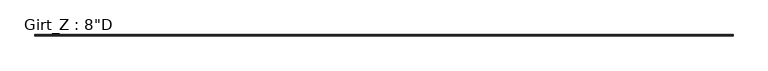
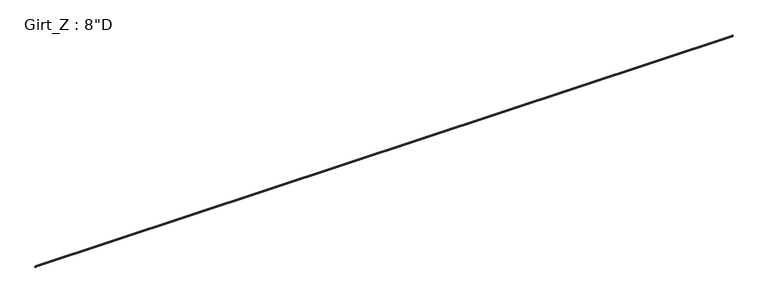
"""IFC4 building model written with IfcOpenShell, lengths in millimetres: beam geometry."""

from ifc_helpers import new_model, si_unit, point, frame, frame_2d, origin, place, context, project, spatial, polyline, circle_curve, trimmed, segment, composite_curve, outline, extrude, source, transform, mapped, element, save


def beam_4e68f0c2(model_context):
    return source(origin(), model_context, "Body", "SweptSolid", [
        extrude(outline(composite_curve([segment(polyline([(-63.5, 101.6), (-3.3734375, 101.6)]), True, "CONTINUOUS"), segment(trimmed(circle_curve(frame_2d((-3.3734375, 96.8375)), 4.7625), [point((-3.3734375, 101.6))], [point((1.3890625, 96.8375))], False, "CARTESIAN"), True, "CONTINUOUS"), segment(polyline([(1.3890625, 96.8375), (1.3890625, -96.8389339)]), True, "CONTINUOUS"), segment(trimmed(circle_curve(frame_2d((3.3748024, -96.8389339)), 1.9857399), [point((1.3890625, -96.8389339))], [point((3.2694106, -98.821875))], True, "CARTESIAN"), True, "CONTINUOUS"), segment(polyline([(3.2694106, -98.821875), (62.204539, -98.821875), (73.6169367, -85.221109), (75.745104, -87.0068534), (63.5, -101.6), (3.3734375, -101.6)]), True, "CONTINUOUS"), segment(trimmed(circle_curve(frame_2d((3.3734375, -96.8375)), 4.7625), [point((3.3734375, -101.6))], [point((-1.3890625, -96.8375))], False, "CARTESIAN"), True, "CONTINUOUS"), segment(polyline([(-1.3890625, -96.8375), (-1.3890625, 96.8381931)]), True, "CONTINUOUS"), segment(trimmed(circle_curve(frame_2d((-3.3741066, 96.8381931)), 1.9850441), [point((-1.3890625, 96.8381931))], [point((-3.3005807, 98.821875))], True, "CARTESIAN"), True, "CONTINUOUS"), segment(polyline([(-3.3005807, 98.821875), (-62.204539, 98.821875), (-73.6169367, 85.221109), (-75.745104, 87.0068534), (-63.5, 101.6)]), True, "CONTINUOUS")], self_intersect=False)), frame((-40615.2697266, 0.0, 0.0), z_axis=(1.0, 0.0, 0.0), x_axis=(0.0, 1.0, 0.0)), (0.0, 0.0, 1.0), 81070.2019531),
    ])


if __name__ == "__main__":
    model = new_model("IFC4")
    model_context = context("Model", 3, world=origin())
    ifc_project = project(units=[si_unit("LENGTHUNIT", "METRE", prefix="MILLI")], contexts=[model_context])
    site = spatial("IfcSite", under=ifc_project)
    building = spatial("IfcBuilding", under=site)
    placement = place(None, origin())
    beam_shape = beam_4e68f0c2(model_context)
    element("IfcBeam", 1, ObjectType="Girt_Z : 8\"D", at=placement, inside=building, context=model_context, shape_type="MappedRepresentation", body=[
        mapped(beam_shape, transform((0.0, 0.0, 0.0), x_axis=(1.0, 0.0, 0.0), y_axis=(0.0, 1.0, 0.0), z_axis=(0.0, 0.0, 1.0))),
    ])
    save(model, "model.ifc")

# Revit data of these elements
# Type "Girt_Z : 8\"D"
#   Web_Thickness = 0' - 0 7/64"
#   Length [instance default] = 10' - 0"
#   Leg_1 = 0' - 2 1/2"
#   Height = 0' - 8"
#   Structural Material [instance default] = none
# Element 1 (IfcBeam, "Girt_Z : 8\"D")
#   Structural Material = Steel
#   Materials on its faces: "Steel"
# Materials
#   "Steel": class "Metal", colour RGB 118 118 114, transparency 0, Description = "Steel, mill finish", Cost = 0
